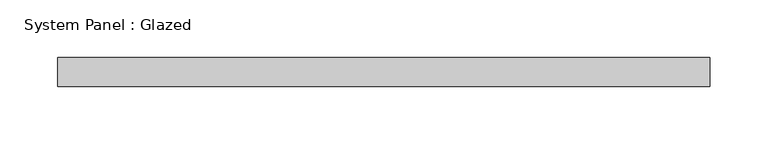
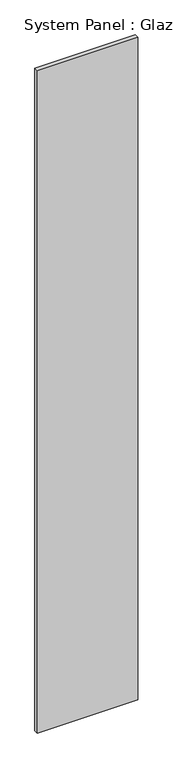
"""IFC4 building model written with IfcOpenShell, lengths in millimetres: plate geometry, System Panel : Glazed."""

from ifc_helpers import new_model, si_unit, origin, origin_with_axes, place, context, project, spatial, polyline, outline, extrude, source, transform, mapped, element, save


def system_panel_glazed_731af6db(model_context):
    return source(origin(), model_context, "Body", "SweptSolid", [
        extrude(outline(polyline([(282.4999998, 24.5), (-282.4999998, 24.5), (-282.4999998, 49.5), (282.4999998, 49.5), (282.4999998, 24.5)])), origin_with_axes(), (0.0, 0.0, 1.0), 3950.0),
    ])


if __name__ == "__main__":
    model = new_model("IFC4")
    model_context = context("Model", 3, world=origin())
    ifc_project = project(units=[si_unit("LENGTHUNIT", "METRE", prefix="MILLI")], contexts=[model_context])
    site = spatial("IfcSite", under=ifc_project)
    building = spatial("IfcBuilding", under=site)
    placement = place(None, origin())
    system_panel_glazed_shape = system_panel_glazed_731af6db(model_context)
    element("IfcPlate", 1, ObjectType="System Panel : Glazed", at=placement, inside=building, context=model_context, shape_type="MappedRepresentation", body=[
        mapped(system_panel_glazed_shape, transform((0.0, 0.0, 0.0), x_axis=(1.0, 0.0, 0.0), y_axis=(0.0, 1.0, 0.0), z_axis=(0.0, 0.0, 1.0))),
    ])
    save(model, "model.ifc")

# Revit data of these elements
# Type "System Panel : Glazed"
#   Keynote = "H11"
#   Construction Type Id = "GSP4R"
#   Analytic Construction = "1/8 in Pilkington single glazing"
#   Visual Light Transmittance = 0.9
#   Solar Heat Gain Coefficient = 0.86
#   Heat Transfer Coefficient (U) = 6.7069 W/(m²·K)
#   Define Thermal Properties by = 1
# Element 1 (IfcPlate, "System Panel : Glazed")
#   Materials on its faces: "Glass"
# Materials
#   "Glass": class "Glass", colour RGB 0 128 192, transparency 0.9, Description = "Soda Lime Glass", Cost = 0
